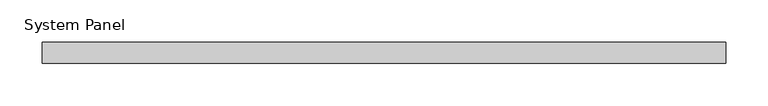
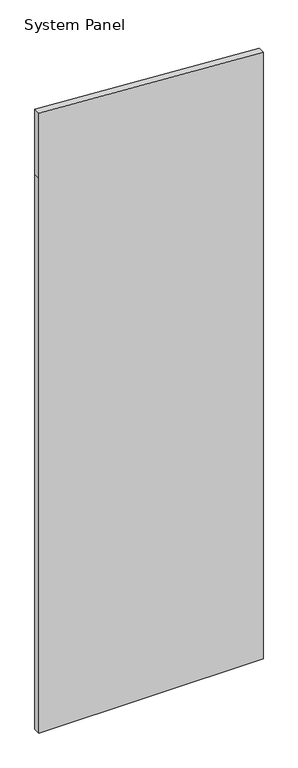
"""IFC4 building model written with IfcOpenShell, lengths in millimetres: plate geometry, System Panel : TEMPERED INSULATED GLAZING (CARDINAL GLASS LoĒ²-240."""

from ifc_helpers import new_model, si_unit, frame, origin, place, context, project, spatial, polyline, outline, extrude, source, transform, mapped, element, save


def system_panel_083ad6d7(model_context):
    return source(origin(), model_context, "Body", "SweptSolid", [
        extrude(outline(polyline([(0.0, -406.5049327), (0.0, 406.5049327), (2127.25, 406.5049327), (2326.7366179, 406.5049327), (2377.5497345, -406.5049327), (2127.25, -406.5049327), (0.0, -406.5049327)])), frame((0.0, 6.35, 0.0), z_axis=(0.0, 1.0, 0.0), x_axis=(0.0, 0.0, 1.0)), (0.0, 0.0, 1.0), 25.4),
    ])


if __name__ == "__main__":
    model = new_model("IFC4")
    model_context = context("Model", 3, world=origin())
    ifc_project = project(units=[si_unit("LENGTHUNIT", "METRE", prefix="MILLI")], contexts=[model_context])
    site = spatial("IfcSite", under=ifc_project)
    building = spatial("IfcBuilding", under=site)
    placement = place(None, origin())
    system_panel_shape = system_panel_083ad6d7(model_context)
    element("IfcPlate", 1, ObjectType="System Panel : TEMPERED INSULATED GLAZING (CARDINAL GLASS LoĒ²-240", at=placement, inside=building, context=model_context, shape_type="MappedRepresentation", body=[
        mapped(system_panel_shape, transform((0.0, 0.0, 0.0), x_axis=(1.0, 0.0, 0.0), y_axis=(0.0, 1.0, 0.0), z_axis=(0.0, 0.0, 1.0))),
    ])
    save(model, "model.ifc")

# Revit data of these elements
# Type "System Panel : TEMPERED INSULATED GLAZING (CARDINAL GLASS LoĒ²-240"
#   Construction Type Id = "opn-s72"
#   Analytic Construction = "Double glazing - 1/4 in thick - low-E/clear (e = 0.1) glass"
#   Visual Light Transmittance = 0.72
#   Solar Heat Gain Coefficient = 0.6
#   Heat Transfer Coefficient (U) = 1.9873 W/(m²·K)
#   Transparency_Hack = 70
# Element 1 (IfcPlate, "System Panel : TEMPERED INSULATED GLAZING (CARDINAL GLASS LoĒ²-240")
#   Materials on its faces: "TEMPERED INSULATED GLAZING (CARDINAL GLASS LoĒ²-240\nOR EQUIVALENT)"
# Materials
#   "TEMPERED INSULATED GLAZING (CARDINAL GLASS LoĒ²-240\nOR EQUIVALENT)": class "Glass", colour RGB 196 205 210, transparency 0.85, Description = "Soda Lime Glass", Cost = 0
